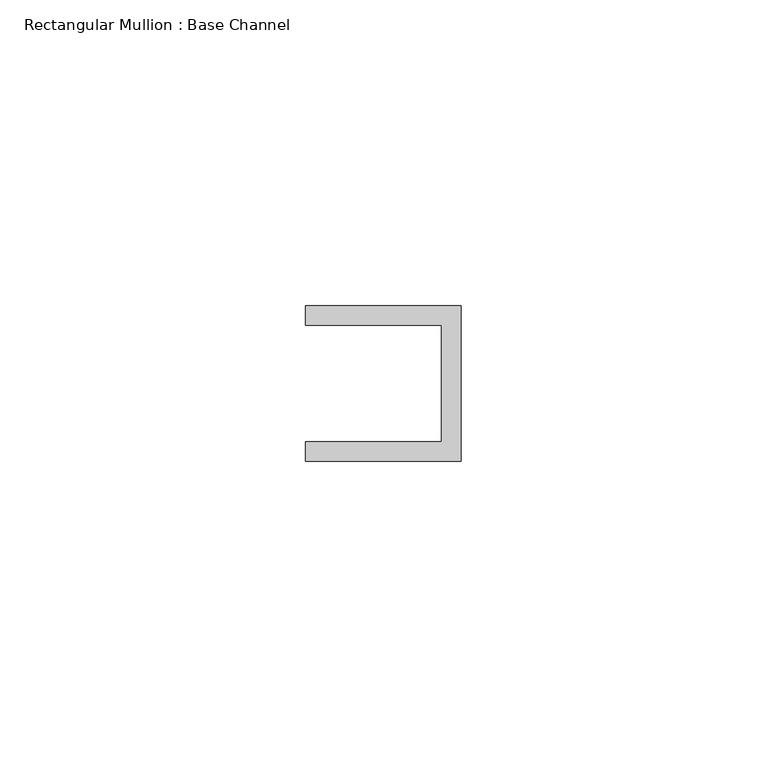
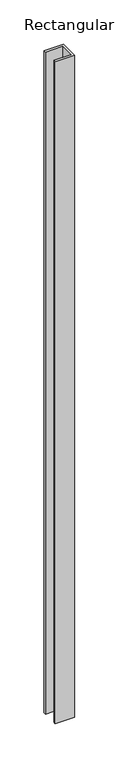
"""IFC4 building model written with IfcOpenShell, lengths in millimetres: member geometry, Rectangular Mullion : Base Channel."""

from ifc_helpers import new_model, si_unit, frame, origin, place, context, project, spatial, polyline, outline, extrude, source, transform, mapped, element, save


def rectangular_mullion_base_channel_4b54669a(model_context):
    return source(origin(), model_context, "Body", "SweptSolid", [
        extrude(outline(polyline([(0.0, -12.7), (-25.4, -12.7), (-25.4, -9.525), (-3.175, -9.525), (-3.175, 9.525), (-25.4, 9.525), (-25.4, 12.7), (0.0, 12.7), (0.0, -12.7)])), frame((0.0, 0.0, -914.4), z_axis=(0.0, 0.0, 1.0), x_axis=(1.0, 0.0, 0.0)), (0.0, 0.0, 1.0), 914.4),
    ])


if __name__ == "__main__":
    model = new_model("IFC4")
    model_context = context("Model", 3, world=origin())
    ifc_project = project(units=[si_unit("LENGTHUNIT", "METRE", prefix="MILLI")], contexts=[model_context])
    site = spatial("IfcSite", under=ifc_project)
    building = spatial("IfcBuilding", under=site)
    placement = place(None, origin())
    rectangular_mullion_base_channel_shape = rectangular_mullion_base_channel_4b54669a(model_context)
    element("IfcMember", 1, ObjectType="Rectangular Mullion : Base Channel", at=placement, inside=building, context=model_context, shape_type="MappedRepresentation", body=[
        mapped(rectangular_mullion_base_channel_shape, transform((0.0, 0.0, 0.0), x_axis=(1.0, 0.0, 0.0), y_axis=(0.0, 1.0, 0.0), z_axis=(0.0, 0.0, 1.0))),
    ])
    save(model, "model.ifc")

# Revit data of these elements
# Type "Rectangular Mullion : Base Channel"
#   built-in parameter 1007322 = 0.0833333 (stored number, unit not read)
#   built-in parameter 1007321 = 0.0416667 (stored number, unit not read)
#   built-in parameter 1007320 = -0.03125 (stored number, unit not read)
# Element 1 (IfcMember, "Rectangular Mullion : Base Channel")
#   Materials on its faces: "ALUM"
# Materials
#   "ALUM": class "Generic", colour RGB 157 157 157, transparency 0, Cost = 0
